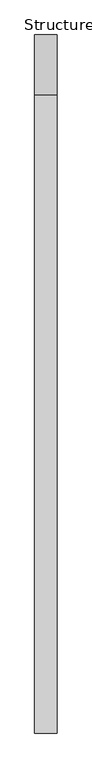
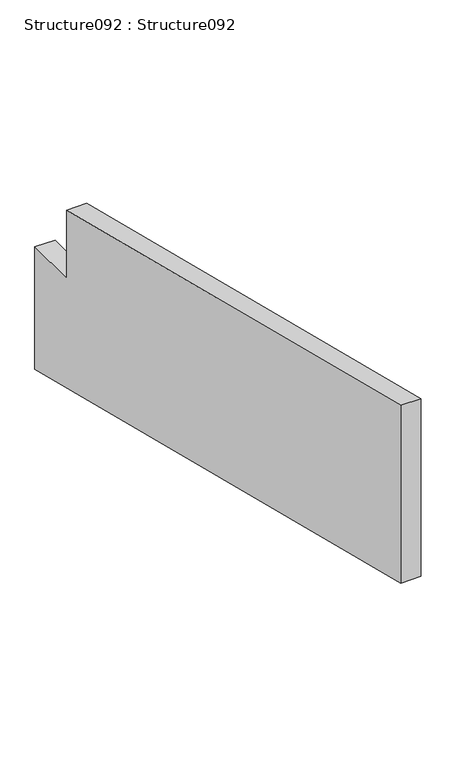
"""IFC4 building model written with IfcOpenShell, lengths in millimetres: proxy geometry, Structure092 : Structure092."""

import ifcopenshell
import ifcopenshell.guid

model = None  # the IFC model being written
_history = None  # IfcOwnerHistory: only IFC2X3 demands one
_inside = {}  # id of a spatial element -> (the spatial element, [elements in it])
_under = {}  # id of a project, library or spatial element -> (it, [spatial elements below it])
_declared = {}  # id of a project -> (the project, [libraries it declares])
_typed = {}  # id of a type object -> (the type object, [elements of that type])
_made_of = {}  # id of a material, layer set ... -> (it, [elements and type objects made of it])


def new_model(schema):
    """Start an empty IFC model of exactly this schema.

    Asked for "IFC4X3", IfcOpenShell would pick the latest addendum, in which some entities
    have other attributes; the version numbers below select the first issue.
    IFC2X3 requires an IfcOwnerHistory on every rooted entity: one is made here for all.
    """
    global model, _history
    if schema == "IFC4X3":
        model = ifcopenshell.file(schema_version=(4, 3, 0, 0))
    else:
        model = ifcopenshell.file(schema=schema)
    _inside.clear()
    _under.clear()
    _declared.clear()
    _typed.clear()
    _made_of.clear()
    _history = None
    if model.schema == "IFC2X3":
        org = make("IfcOrganization", Name="unknown")
        user = make(
            "IfcPersonAndOrganization",
            ThePerson=make("IfcPerson", FamilyName="unknown"),
            TheOrganization=org,
        )
        app = make(
            "IfcApplication",
            ApplicationDeveloper=org,
            Version="unknown",
            ApplicationFullName="unknown",
            ApplicationIdentifier="unknown",
        )
        _history = make(
            "IfcOwnerHistory",
            OwningUser=user,
            OwningApplication=app,
            ChangeAction="ADDED",
            CreationDate=0,
        )
    return model


def make(cls, **values):
    """One entity of the class cls with the attributes given. An attribute that is None is left unset."""
    return model.create_entity(
        cls, **{name: value for name, value in values.items() if value is not None}
    )


def rooted(cls, **values):
    """An entity with a GlobalId (a new one), such as an element, a storey or a relation."""
    return make(cls, GlobalId=ifcopenshell.guid.new(), OwnerHistory=_history, **values)


def si_unit(unit_type, name, prefix=None):
    """IfcSIUnit, for example si_unit("LENGTHUNIT", "METRE", prefix="MILLI")."""
    return make("IfcSIUnit", UnitType=unit_type, Prefix=prefix, Name=name)


def assignment(units):
    """IfcUnitAssignment: the units of a project."""
    return None if units is None else make("IfcUnitAssignment", Units=units)


def point(xyz):
    """IfcCartesianPoint."""
    return None if xyz is None else make("IfcCartesianPoint", Coordinates=xyz)


def direction(xyz):
    """IfcDirection."""
    return None if xyz is None else make("IfcDirection", DirectionRatios=xyz)


def frame(location, z_axis=None, x_axis=None):
    """IfcAxis2Placement3D, a coordinate frame: its origin and axes. An axis left out is left unset."""
    return make(
        "IfcAxis2Placement3D",
        Location=point(location),
        Axis=direction(z_axis),
        RefDirection=direction(x_axis),
    )


def origin():
    """The frame at (0, 0, 0) with its axes left unset."""
    return frame((0.0, 0.0, 0.0))


def place(relative_to, where):
    """IfcLocalPlacement: puts the frame where relative to a parent placement (None: the world)."""
    return make(
        "IfcLocalPlacement", PlacementRelTo=relative_to, RelativePlacement=where
    )


def context(
    kind, dimensions, precision=None, world=None, true_north=None, identifier=None
):
    """IfcGeometricRepresentationContext, for example the 3D "Model" context."""
    return make(
        "IfcGeometricRepresentationContext",
        ContextIdentifier=identifier,
        ContextType=kind,
        CoordinateSpaceDimension=dimensions,
        Precision=precision,
        WorldCoordinateSystem=world,
        TrueNorth=true_north,
    )


def project(units=None, contexts=None):
    """IfcProject with its units and contexts."""
    return rooted(
        "IfcProject",
        Name="project",
        RepresentationContexts=contexts,
        UnitsInContext=assignment(units),
    )


def spatial(cls, under=None, at=None, **own):
    """A site, building, storey or space (cls), placed at a placement, below another one or the project."""
    s = rooted(cls, ObjectPlacement=at, **own)
    if under is not None:
        _under.setdefault(under.id(), (under, []))[1].append(s)
    return s


def polyline(points):
    """IfcPolyline through the points."""
    return make("IfcPolyline", Points=[point(p) for p in points])


def outline(outer, holes=None, kind="AREA"):
    """IfcArbitraryClosedProfileDef: a profile drawn as a closed curve; with holes, ...WithVoids."""
    if holes is None:
        return make("IfcArbitraryClosedProfileDef", ProfileType=kind, OuterCurve=outer)
    return make(
        "IfcArbitraryProfileDefWithVoids",
        ProfileType=kind,
        OuterCurve=outer,
        InnerCurves=holes,
    )


def extrude(swept, where, along, depth):
    """IfcExtrudedAreaSolid: the profile swept, set in the frame where, extruded along a direction by depth."""
    return make(
        "IfcExtrudedAreaSolid",
        SweptArea=swept,
        Position=where,
        ExtrudedDirection=direction(along),
        Depth=depth,
    )


def shape(context_of_items, identifier, shape_type, items):
    """IfcShapeRepresentation: the items that make up one representation, for example the "Body"."""
    return make(
        "IfcShapeRepresentation",
        ContextOfItems=context_of_items,
        RepresentationIdentifier=identifier,
        RepresentationType=shape_type,
        Items=items,
    )


def source(mapping_origin, context_of_items, identifier, shape_type, items):
    """IfcRepresentationMap: a shape defined once, which mapped items show again and again."""
    return make(
        "IfcRepresentationMap",
        MappingOrigin=mapping_origin,
        MappedRepresentation=shape(context_of_items, identifier, shape_type, items),
    )


def transform(
    local_origin,
    x_axis=None,
    y_axis=None,
    z_axis=None,
    scale=None,
    scale2=None,
    scale3=None,
    uniform=True,
):
    """IfcCartesianTransformationOperator3D, or its non-uniform kind. x_axis, y_axis, z_axis: its Axis1, 2, 3."""
    if uniform:
        return make(
            "IfcCartesianTransformationOperator3D",
            Axis1=direction(x_axis),
            Axis2=direction(y_axis),
            LocalOrigin=point(local_origin),
            Scale=scale,
            Axis3=direction(z_axis),
        )
    return make(
        "IfcCartesianTransformationOperator3DnonUniform",
        Axis1=direction(x_axis),
        Axis2=direction(y_axis),
        LocalOrigin=point(local_origin),
        Scale=scale,
        Axis3=direction(z_axis),
        Scale2=scale2,
        Scale3=scale3,
    )


def mapped(mapping_source, mapping_target):
    """IfcMappedItem: shows the shape of a source again, moved by a transform."""
    return make(
        "IfcMappedItem", MappingSource=mapping_source, MappingTarget=mapping_target
    )


def made_of(thing, what):
    """Note that an element or type object is made of a material, layer set ...; save() writes the relation."""
    if what is not None:
        _made_of.setdefault(what.id(), (what, []))[1].append(thing)
    return thing


def element(
    cls,
    number,
    at=None,
    inside=None,
    cuts=None,
    type_object=None,
    material=None,
    context=None,
    identifier="Body",
    shape_type=None,
    held_by="IfcProductDefinitionShape",
    body=None,
    shapes=None,
    **own,
):
    """One element of the class cls, such as IfcWall. Its Tag is "e" and its number.

    at: its placement. inside: the storey or other place that contains it. cuts: it is an
    opening in that element (IfcRelVoidsElement). A single representation is given by context,
    identifier, shape_type and body (its items); several are given by shapes. held_by: the class
    of the entity that holds the representations. save() writes the other relations.
    """
    e = rooted(cls, Tag="e%d" % number, ObjectPlacement=at, **own)
    if body is not None:
        shapes = [shape(context, identifier, shape_type, body)]
    if shapes is not None:
        e.Representation = make(held_by, Representations=shapes)
    if inside is not None:
        _inside.setdefault(inside.id(), (inside, []))[1].append(e)
    if cuts is not None:
        rooted(
            "IfcRelVoidsElement", RelatingBuildingElement=cuts, RelatedOpeningElement=e
        )
    if type_object is not None:
        _typed.setdefault(type_object.id(), (type_object, []))[1].append(e)
    return made_of(e, material)


def aggregate(whole, parts):
    """IfcRelAggregates: a whole, such as a stair, and the parts it consists of."""
    return rooted("IfcRelAggregates", RelatingObject=whole, RelatedObjects=parts)


def save(model, path):
    """Write the relations noted so far, then the file.

    IfcRelAggregates (storeys below a building ...), IfcRelContainedInSpatialStructure (elements
    in a storey), IfcRelDefinesByType, IfcRelAssociatesMaterial and IfcRelDeclares: one each for
    every whole, place, type object, material and project.
    """
    for whole, parts in _under.values():
        aggregate(whole, parts)
    for where, things in _inside.values():
        rooted(
            "IfcRelContainedInSpatialStructure",
            RelatedElements=things,
            RelatingStructure=where,
        )
    for kind, things in _typed.values():
        rooted("IfcRelDefinesByType", RelatedObjects=things, RelatingType=kind)
    for what, things in _made_of.values():
        rooted("IfcRelAssociatesMaterial", RelatedObjects=things, RelatingMaterial=what)
    for by, libraries in _declared.values():
        rooted("IfcRelDeclares", RelatingContext=by, RelatedDefinitions=libraries)
    model.write(path)


def structure092_structure092_623fca83(model_context):
    return source(origin(), model_context, "Body", "SweptSolid", [
        extrude(outline(polyline([(3064.1094171, 41796.3564587), (4341.2980909, 41477.0623881), (4341.2980909, 41318.4021881), (4461.9480928, 41318.4021881), (4461.9480928, 41032.8236949), (3064.1094171, 41382.2833638), (3064.1094171, 41796.3564587)])), frame((1007.8867446, 0.0, 0.0), z_axis=(1.0, 0.0, 0.0), x_axis=(0.0, 1.0, 0.0)), (0.0, 0.0, 1.0), 44.45),
    ])


if __name__ == "__main__":
    model = new_model("IFC4")
    model_context = context("Model", 3, world=origin())
    ifc_project = project(units=[si_unit("LENGTHUNIT", "METRE", prefix="MILLI")], contexts=[model_context])
    site = spatial("IfcSite", under=ifc_project)
    building = spatial("IfcBuilding", under=site)
    placement = place(None, origin())
    structure092_structure092_shape = structure092_structure092_623fca83(model_context)
    element("IfcBuildingElementProxy", 1, Name="Structure092 : Structure092", ObjectType="Structure092 : Structure092", at=placement, inside=building, context=model_context, shape_type="MappedRepresentation", body=[
        mapped(structure092_structure092_shape, transform((0.0, 0.0, 0.0), x_axis=(1.0, 0.0, 0.0), y_axis=(0.0, 1.0, 0.0), z_axis=(0.0, 0.0, 1.0))),
    ])
    save(model, "model.ifc")

# Revit data of these elements
# Type "Structure092 : Structure092"
#   NameOverride = "Structure092"
# Element 1 (IfcBuildingElementProxy, "Structure092 : Structure092")
#   Materials on its faces: "STRUCTURAL MEMBER (SEE DWGS)"
# Materials
#   "STRUCTURAL MEMBER (SEE DWGS)": class "Unassigned", colour RGB 214 178 158, transparency 0, Cost = 0
